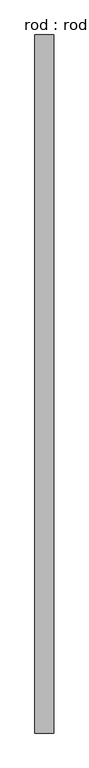
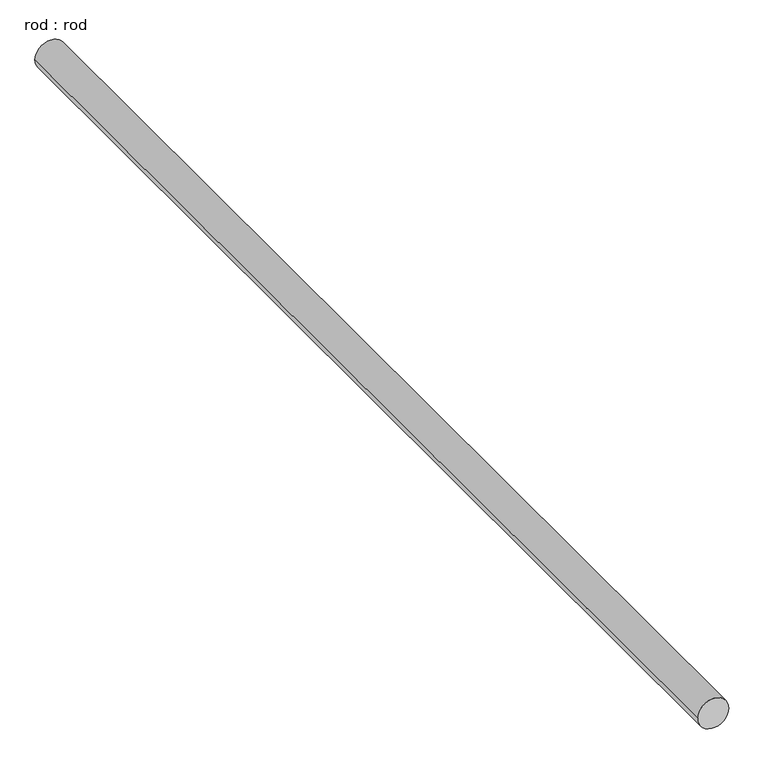
"""IFC4 building model written with IfcOpenShell, lengths in millimetres: proxy geometry, rod : rod."""

from ifc_helpers import new_model, si_unit, point, frame, frame_2d, origin, place, context, project, spatial, circle_curve, trimmed, segment, composite_curve, outline, extrude, source, transform, mapped, element, save


def rod_rod_bf01b327(model_context):
    return source(origin(), model_context, "Body", "SweptSolid", [
        extrude(outline(composite_curve([segment(trimmed(circle_curve(frame_2d((0.0108462, 0.0)), 200.0), [point((0.0108462, 200.0))], [point((0.0108462, -200.0))], False, "CARTESIAN"), True, "CONTINUOUS"), segment(trimmed(circle_curve(frame_2d((0.0108462, 0.0)), 200.0), [point((0.0108462, -200.0))], [point((0.0108462, 200.0))], False, "CARTESIAN"), True, "CONTINUOUS")], self_intersect=False)), frame((0.0, -3282.2713847, 0.0), z_axis=(0.0, 1.0, 0.0), x_axis=(0.0, 0.0, 1.0)), (0.0, 0.0, 1.0), 14750.0),
    ])


if __name__ == "__main__":
    model = new_model("IFC4")
    model_context = context("Model", 3, world=origin())
    ifc_project = project(units=[si_unit("LENGTHUNIT", "METRE", prefix="MILLI")], contexts=[model_context])
    site = spatial("IfcSite", under=ifc_project)
    building = spatial("IfcBuilding", under=site)
    placement = place(None, origin())
    rod_rod_shape = rod_rod_bf01b327(model_context)
    element("IfcBuildingElementProxy", 1, Name="rod : rod", ObjectType="rod : rod", at=placement, inside=building, context=model_context, shape_type="MappedRepresentation", body=[
        mapped(rod_rod_shape, transform((0.0, 0.0, 0.0), x_axis=(1.0, 0.0, 0.0), y_axis=(0.0, 1.0, 0.0), z_axis=(0.0, 0.0, 1.0))),
    ])
    save(model, "model.ifc")

# Revit data of these elements
# Type "rod : rod"
#   Default Elevation = 0
